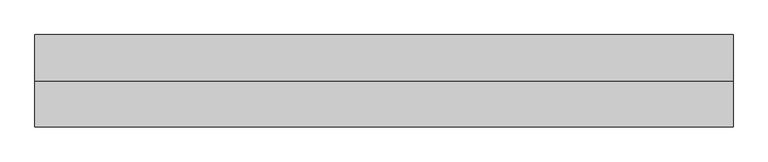
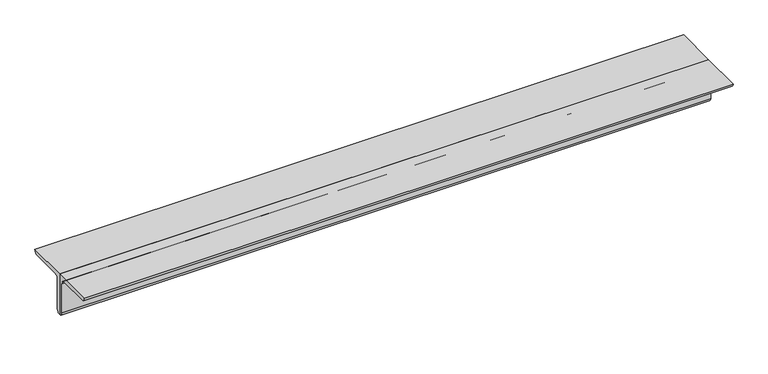
"""IFC4 building model written with IfcOpenShell, lengths in millimetres: beam geometry, 0123_Steel Framing_2Ls-KSD3502 : H_SB_AR_S04_2Ls-130x130x12_VBR1."""

import ifcopenshell
import ifcopenshell.guid

model = None  # the IFC model being written
_history = None  # IfcOwnerHistory: only IFC2X3 demands one
_inside = {}  # id of a spatial element -> (the spatial element, [elements in it])
_under = {}  # id of a project, library or spatial element -> (it, [spatial elements below it])
_declared = {}  # id of a project -> (the project, [libraries it declares])
_typed = {}  # id of a type object -> (the type object, [elements of that type])
_made_of = {}  # id of a material, layer set ... -> (it, [elements and type objects made of it])


def new_model(schema):
    """Start an empty IFC model of exactly this schema.

    Asked for "IFC4X3", IfcOpenShell would pick the latest addendum, in which some entities
    have other attributes; the version numbers below select the first issue.
    IFC2X3 requires an IfcOwnerHistory on every rooted entity: one is made here for all.
    """
    global model, _history
    if schema == "IFC4X3":
        model = ifcopenshell.file(schema_version=(4, 3, 0, 0))
    else:
        model = ifcopenshell.file(schema=schema)
    _inside.clear()
    _under.clear()
    _declared.clear()
    _typed.clear()
    _made_of.clear()
    _history = None
    if model.schema == "IFC2X3":
        org = make("IfcOrganization", Name="unknown")
        user = make(
            "IfcPersonAndOrganization",
            ThePerson=make("IfcPerson", FamilyName="unknown"),
            TheOrganization=org,
        )
        app = make(
            "IfcApplication",
            ApplicationDeveloper=org,
            Version="unknown",
            ApplicationFullName="unknown",
            ApplicationIdentifier="unknown",
        )
        _history = make(
            "IfcOwnerHistory",
            OwningUser=user,
            OwningApplication=app,
            ChangeAction="ADDED",
            CreationDate=0,
        )
    return model


def make(cls, **values):
    """One entity of the class cls with the attributes given. An attribute that is None is left unset."""
    return model.create_entity(
        cls, **{name: value for name, value in values.items() if value is not None}
    )


def rooted(cls, **values):
    """An entity with a GlobalId (a new one), such as an element, a storey or a relation."""
    return make(cls, GlobalId=ifcopenshell.guid.new(), OwnerHistory=_history, **values)


def si_unit(unit_type, name, prefix=None):
    """IfcSIUnit, for example si_unit("LENGTHUNIT", "METRE", prefix="MILLI")."""
    return make("IfcSIUnit", UnitType=unit_type, Prefix=prefix, Name=name)


def assignment(units):
    """IfcUnitAssignment: the units of a project."""
    return None if units is None else make("IfcUnitAssignment", Units=units)


def point(xyz):
    """IfcCartesianPoint."""
    return None if xyz is None else make("IfcCartesianPoint", Coordinates=xyz)


def direction(xyz):
    """IfcDirection."""
    return None if xyz is None else make("IfcDirection", DirectionRatios=xyz)


def frame(location, z_axis=None, x_axis=None):
    """IfcAxis2Placement3D, a coordinate frame: its origin and axes. An axis left out is left unset."""
    return make(
        "IfcAxis2Placement3D",
        Location=point(location),
        Axis=direction(z_axis),
        RefDirection=direction(x_axis),
    )


def frame_2d(location, x_axis=None):
    """IfcAxis2Placement2D, a coordinate frame in the plane: its origin and x axis."""
    return make(
        "IfcAxis2Placement2D", Location=point(location), RefDirection=direction(x_axis)
    )


def origin():
    """The frame at (0, 0, 0) with its axes left unset."""
    return frame((0.0, 0.0, 0.0))


def place(relative_to, where):
    """IfcLocalPlacement: puts the frame where relative to a parent placement (None: the world)."""
    return make(
        "IfcLocalPlacement", PlacementRelTo=relative_to, RelativePlacement=where
    )


def context(
    kind, dimensions, precision=None, world=None, true_north=None, identifier=None
):
    """IfcGeometricRepresentationContext, for example the 3D "Model" context."""
    return make(
        "IfcGeometricRepresentationContext",
        ContextIdentifier=identifier,
        ContextType=kind,
        CoordinateSpaceDimension=dimensions,
        Precision=precision,
        WorldCoordinateSystem=world,
        TrueNorth=true_north,
    )


def project(units=None, contexts=None):
    """IfcProject with its units and contexts."""
    return rooted(
        "IfcProject",
        Name="project",
        RepresentationContexts=contexts,
        UnitsInContext=assignment(units),
    )


def spatial(cls, under=None, at=None, **own):
    """A site, building, storey or space (cls), placed at a placement, below another one or the project."""
    s = rooted(cls, ObjectPlacement=at, **own)
    if under is not None:
        _under.setdefault(under.id(), (under, []))[1].append(s)
    return s


def polyline(points):
    """IfcPolyline through the points."""
    return make("IfcPolyline", Points=[point(p) for p in points])


def circle_curve(where, radius):
    """IfcCircle in the frame where."""
    return make("IfcCircle", Position=where, Radius=radius)


def trimmed(basis, trim1, trim2, sense, master):
    """IfcTrimmedCurve: the piece of a basis curve between two trims."""
    return make(
        "IfcTrimmedCurve",
        BasisCurve=basis,
        Trim1=trim1,
        Trim2=trim2,
        SenseAgreement=sense,
        MasterRepresentation=master,
    )


def segment(curve, same_sense, transition):
    """IfcCompositeCurveSegment."""
    return make(
        "IfcCompositeCurveSegment",
        Transition=transition,
        SameSense=same_sense,
        ParentCurve=curve,
    )


def composite_curve(segments, self_intersect=None):
    """IfcCompositeCurve: segments joined end to end."""
    return make("IfcCompositeCurve", Segments=segments, SelfIntersect=self_intersect)


def outline(outer, holes=None, kind="AREA"):
    """IfcArbitraryClosedProfileDef: a profile drawn as a closed curve; with holes, ...WithVoids."""
    if holes is None:
        return make("IfcArbitraryClosedProfileDef", ProfileType=kind, OuterCurve=outer)
    return make(
        "IfcArbitraryProfileDefWithVoids",
        ProfileType=kind,
        OuterCurve=outer,
        InnerCurves=holes,
    )


def extrude(swept, where, along, depth):
    """IfcExtrudedAreaSolid: the profile swept, set in the frame where, extruded along a direction by depth."""
    return make(
        "IfcExtrudedAreaSolid",
        SweptArea=swept,
        Position=where,
        ExtrudedDirection=direction(along),
        Depth=depth,
    )


def shape(context_of_items, identifier, shape_type, items):
    """IfcShapeRepresentation: the items that make up one representation, for example the "Body"."""
    return make(
        "IfcShapeRepresentation",
        ContextOfItems=context_of_items,
        RepresentationIdentifier=identifier,
        RepresentationType=shape_type,
        Items=items,
    )


def source(mapping_origin, context_of_items, identifier, shape_type, items):
    """IfcRepresentationMap: a shape defined once, which mapped items show again and again."""
    return make(
        "IfcRepresentationMap",
        MappingOrigin=mapping_origin,
        MappedRepresentation=shape(context_of_items, identifier, shape_type, items),
    )


def transform(
    local_origin,
    x_axis=None,
    y_axis=None,
    z_axis=None,
    scale=None,
    scale2=None,
    scale3=None,
    uniform=True,
):
    """IfcCartesianTransformationOperator3D, or its non-uniform kind. x_axis, y_axis, z_axis: its Axis1, 2, 3."""
    if uniform:
        return make(
            "IfcCartesianTransformationOperator3D",
            Axis1=direction(x_axis),
            Axis2=direction(y_axis),
            LocalOrigin=point(local_origin),
            Scale=scale,
            Axis3=direction(z_axis),
        )
    return make(
        "IfcCartesianTransformationOperator3DnonUniform",
        Axis1=direction(x_axis),
        Axis2=direction(y_axis),
        LocalOrigin=point(local_origin),
        Scale=scale,
        Axis3=direction(z_axis),
        Scale2=scale2,
        Scale3=scale3,
    )


def mapped(mapping_source, mapping_target):
    """IfcMappedItem: shows the shape of a source again, moved by a transform."""
    return make(
        "IfcMappedItem", MappingSource=mapping_source, MappingTarget=mapping_target
    )


def made_of(thing, what):
    """Note that an element or type object is made of a material, layer set ...; save() writes the relation."""
    if what is not None:
        _made_of.setdefault(what.id(), (what, []))[1].append(thing)
    return thing


def element(
    cls,
    number,
    at=None,
    inside=None,
    cuts=None,
    type_object=None,
    material=None,
    context=None,
    identifier="Body",
    shape_type=None,
    held_by="IfcProductDefinitionShape",
    body=None,
    shapes=None,
    **own,
):
    """One element of the class cls, such as IfcWall. Its Tag is "e" and its number.

    at: its placement. inside: the storey or other place that contains it. cuts: it is an
    opening in that element (IfcRelVoidsElement). A single representation is given by context,
    identifier, shape_type and body (its items); several are given by shapes. held_by: the class
    of the entity that holds the representations. save() writes the other relations.
    """
    e = rooted(cls, Tag="e%d" % number, ObjectPlacement=at, **own)
    if body is not None:
        shapes = [shape(context, identifier, shape_type, body)]
    if shapes is not None:
        e.Representation = make(held_by, Representations=shapes)
    if inside is not None:
        _inside.setdefault(inside.id(), (inside, []))[1].append(e)
    if cuts is not None:
        rooted(
            "IfcRelVoidsElement", RelatingBuildingElement=cuts, RelatedOpeningElement=e
        )
    if type_object is not None:
        _typed.setdefault(type_object.id(), (type_object, []))[1].append(e)
    return made_of(e, material)


def aggregate(whole, parts):
    """IfcRelAggregates: a whole, such as a stair, and the parts it consists of."""
    return rooted("IfcRelAggregates", RelatingObject=whole, RelatedObjects=parts)


def save(model, path):
    """Write the relations noted so far, then the file.

    IfcRelAggregates (storeys below a building ...), IfcRelContainedInSpatialStructure (elements
    in a storey), IfcRelDefinesByType, IfcRelAssociatesMaterial and IfcRelDeclares: one each for
    every whole, place, type object, material and project.
    """
    for whole, parts in _under.values():
        aggregate(whole, parts)
    for where, things in _inside.values():
        rooted(
            "IfcRelContainedInSpatialStructure",
            RelatedElements=things,
            RelatingStructure=where,
        )
    for kind, things in _typed.values():
        rooted("IfcRelDefinesByType", RelatedObjects=things, RelatingType=kind)
    for what, things in _made_of.values():
        rooted("IfcRelAssociatesMaterial", RelatedObjects=things, RelatingMaterial=what)
    for by, libraries in _declared.values():
        rooted("IfcRelDeclares", RelatingContext=by, RelatedDefinitions=libraries)
    model.write(path)


def beam_d0207f13(model_context):
    return source(origin(), model_context, "Body", "SweptSolid", [
        extrude(outline(composite_curve([segment(polyline([(0.0, 36.4), (130.0, 36.4)]), True, "CONTINUOUS"), segment(trimmed(circle_curve(frame_2d((118.0, 36.4)), 12.0), [point((130.0, 36.4))], [point((118.0, 24.4))], False, "CARTESIAN"), True, "CONTINUOUS"), segment(polyline([(118.0, 24.4), (24.0, 24.4)]), True, "CONTINUOUS"), segment(trimmed(circle_curve(frame_2d((24.0, 12.4)), 12.0), [point((24.0, 24.4))], [point((12.0, 12.4))], True, "CARTESIAN"), True, "CONTINUOUS"), segment(polyline([(12.0, 12.4), (12.0, -81.6)]), True, "CONTINUOUS"), segment(trimmed(circle_curve(frame_2d((0.0, -81.6)), 12.0), [point((12.0, -81.6))], [point((0.0, -93.6))], False, "CARTESIAN"), True, "CONTINUOUS"), segment(polyline([(0.0, -93.6), (0.0, 36.4)]), True, "CONTINUOUS")], self_intersect=False)), frame((-1052.8208184, 0.0, 0.0), z_axis=(1.0, 0.0, 0.0), x_axis=(0.0, 1.0, 0.0)), (0.0, 0.0, 1.0), 1965.6424176),
        extrude(outline(composite_curve([segment(polyline([(0.0, 36.4), (0.0, -93.6)]), True, "CONTINUOUS"), segment(trimmed(circle_curve(frame_2d((0.0, -81.6)), 12.0), [point((0.0, -93.6))], [point((-12.0, -81.6))], False, "CARTESIAN"), True, "CONTINUOUS"), segment(polyline([(-12.0, -81.6), (-12.0, 12.4)]), True, "CONTINUOUS"), segment(trimmed(circle_curve(frame_2d((-24.0, 12.4)), 12.0), [point((-12.0, 12.4))], [point((-24.0, 24.4))], True, "CARTESIAN"), True, "CONTINUOUS"), segment(polyline([(-24.0, 24.4), (-118.0, 24.4)]), True, "CONTINUOUS"), segment(trimmed(circle_curve(frame_2d((-118.0, 36.4)), 12.0), [point((-118.0, 24.4))], [point((-130.0, 36.4))], False, "CARTESIAN"), True, "CONTINUOUS"), segment(polyline([(-130.0, 36.4), (0.0, 36.4)]), True, "CONTINUOUS")], self_intersect=False)), frame((-1052.8208184, 0.0, 0.0), z_axis=(1.0, 0.0, 0.0), x_axis=(0.0, 1.0, 0.0)), (0.0, 0.0, 1.0), 1965.6424176),
    ])


if __name__ == "__main__":
    model = new_model("IFC4")
    model_context = context("Model", 3, world=origin())
    ifc_project = project(units=[si_unit("LENGTHUNIT", "METRE", prefix="MILLI")], contexts=[model_context])
    site = spatial("IfcSite", under=ifc_project)
    building = spatial("IfcBuilding", under=site)
    placement = place(None, origin())
    beam_shape = beam_d0207f13(model_context)
    element("IfcBeam", 1, ObjectType="0123_Steel Framing_2Ls-KSD3502 : H_SB_AR_S04_2Ls-130x130x12_VBR1", at=placement, inside=building, context=model_context, shape_type="MappedRepresentation", body=[
        mapped(beam_shape, transform((0.0, 0.0, 0.0), x_axis=(1.0, 0.0, 0.0), y_axis=(0.0, 1.0, 0.0), z_axis=(0.0, 0.0, 1.0))),
    ])
    save(model, "model.ifc")

# Revit data of these elements
# Type "0123_Steel Framing_2Ls-KSD3502 : H_SB_AR_S04_2Ls-130x130x12_VBR1"
#   Type Mark = "VBR1"
#   Assembly Code = "B10"
#   Legs = "SLBB"
#   W = 8.97
#   Perimeter = 1.04 m²/m
#   Nominal Weight = 46.80 kgf/m
#   Length [instance default] = 1000 mm
#   Space = 0 mm
#   b = 130 mm
#   d = 130 mm
#   t = 12 mm
#   y = 36.4 mm
#   A = 0.005952 m²
#   Structural Material [instance default] = Steel ASTM A36
# Element 1 (IfcBeam, "0123_Steel Framing_2Ls-KSD3502 : H_SB_AR_S04_2Ls-130x130x12_VBR1")
#   Materials on its faces: "Steel ASTM A36"
# Materials
#   "Steel ASTM A36": class "Metal", colour RGB 199 199 199, transparency 0, Description = "Structural steel, ASTM A36 Grade B, mill finish", Cost = 0
